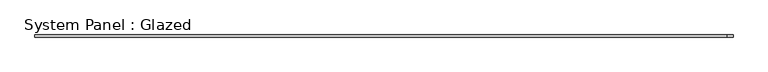
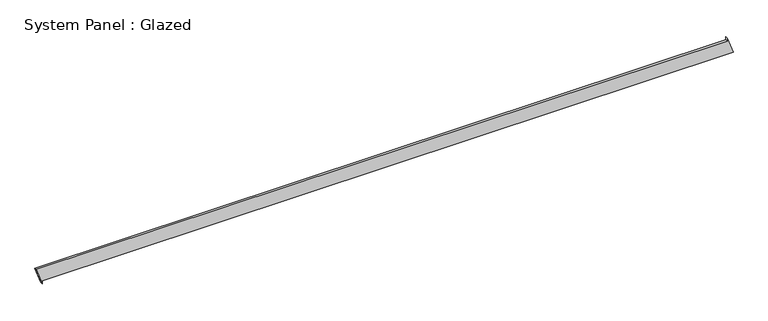
"""IFC4 building model written with IfcOpenShell, lengths in millimetres: plate geometry, System Panel : Glazed."""

from ifc_helpers import new_model, si_unit, frame, origin, place, context, project, spatial, polyline, outline, extrude, source, transform, mapped, element, save


def system_panel_glazed_df643311(model_context):
    return source(origin(), model_context, "Body", "SweptSolid", [
        extrude(outline(polyline([(0.0, -3958.3728013), (35.3553391, -3958.3728013), (35.3553391, 4028.0187252), (234.3660482, 3958.4192766), (199.0107092, 3958.4193631), (198.9911695, -4028.0187252), (0.0, -3958.3728013)])), frame((0.0, -49.5, 0.0), z_axis=(0.0, 1.0, 0.0), x_axis=(0.0, 0.0, 1.0)), (0.0, 0.0, 1.0), 25.0),
    ])


if __name__ == "__main__":
    model = new_model("IFC4")
    model_context = context("Model", 3, world=origin())
    ifc_project = project(units=[si_unit("LENGTHUNIT", "METRE", prefix="MILLI")], contexts=[model_context])
    site = spatial("IfcSite", under=ifc_project)
    building = spatial("IfcBuilding", under=site)
    placement = place(None, origin())
    system_panel_glazed_shape = system_panel_glazed_df643311(model_context)
    element("IfcPlate", 1, ObjectType="System Panel : Glazed", at=placement, inside=building, context=model_context, shape_type="MappedRepresentation", body=[
        mapped(system_panel_glazed_shape, transform((0.0, 0.0, 0.0), x_axis=(1.0, 0.0, 0.0), y_axis=(0.0, 1.0, 0.0), z_axis=(0.0, 0.0, 1.0))),
    ])
    save(model, "model.ifc")

# Revit data of these elements
# Element 1 (IfcPlate, "System Panel : Glazed")
#   Materials on its faces: "Glass"
# Materials
#   "Glass": class "Glass", colour RGB 218 227 224, transparency 0.85, Description = "Soda Lime Glass", Cost = 0
